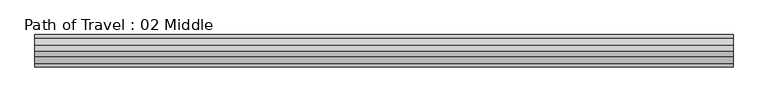
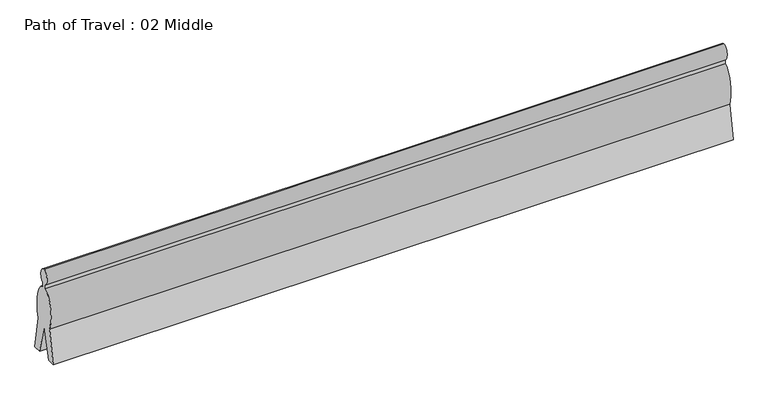
"""IFC4 building model written with IfcOpenShell, lengths in millimetres: proxy geometry, Path of Travel : 02 Middle."""

from ifc_helpers import new_model, si_unit, point, frame, origin, place, context, project, spatial, ellipse_curve, trimmed, source, transform, mapped, element, save
from ifc_brep_helpers import plane_surface, extruded_surface, advanced_brep


def path_of_travel_02_middle_47484a08(model_context):
    return source(origin(), model_context, "Body", "AdvancedBrep", [
        advanced_brep(
        [(227.5554837, 0.0, 1727.2), (227.5554837, 42.9018657, 1436.6534209), (227.5554837, 42.9018657, 1363.4763406), (227.5554837, 184.1186263, 643.4144547), (227.5554837, 297.5699544, 0.0), (227.5554837, 145.6574193, 0.0), (227.5554837, 0.0, 584.2), (227.5554837, -145.6574193, 0.0), (227.5554837, -297.5699544, 0.0), (227.5554837, -184.1186263, 643.4144547), (227.5554837, -42.9018657, 1363.4763406), (227.5554837, -42.9018657, 1436.6534209), (13029.1554837, 0.0, 1727.2), (13029.1554837, -42.9018657, 1436.6534209), (13029.1554837, -42.9018657, 1363.4763406), (13029.1554837, -184.1186263, 643.4144547), (13029.1554837, -297.5699544, 0.0), (13029.1554837, -145.6574193, 0.0), (13029.1554837, 0.0, 584.2), (13029.1554837, 145.6574193, 0.0), (13029.1554837, 297.5699544, 0.0), (13029.1554837, 184.1186263, 643.4144547), (13029.1554837, 42.9018657, 1363.4763406), (13029.1554837, 42.9018657, 1436.6534209)],
        [
            (0, 1, ellipse_curve(frame((227.5554837, 0.0, 1574.8), z_axis=(-1.0, 0.0, 0.0), x_axis=(0.0, 0.0, 1.0)), 152.4, 101.6)),
            (1, 2),
            (2, 3, ellipse_curve(frame((227.5554837, 0.0, 914.4), z_axis=(-1.0, 0.0, 0.0), x_axis=(0.0, 0.0, -1.0)), 457.2, 228.6)),
            (3, 4),
            (4, 5),
            (5, 6),
            (6, 7),
            (7, 8),
            (8, 9),
            (9, 10, ellipse_curve(frame((227.5554837, 0.0, 914.4), z_axis=(-1.0, 0.0, 0.0), x_axis=(0.0, 0.0, -1.0)), 457.2, 228.6)),
            (10, 11),
            (11, 0, ellipse_curve(frame((227.5554837, 0.0, 1574.8), z_axis=(-1.0, 0.0, 0.0), x_axis=(0.0, 0.0, 1.0)), 152.4, 101.6)),
            (12, 13, ellipse_curve(frame((13029.1554837, 0.0, 1574.8), z_axis=(1.0, 0.0, 0.0), x_axis=(0.0, 0.0, 1.0)), 152.4, 101.6)),
            (13, 14),
            (14, 15, ellipse_curve(frame((13029.1554837, 0.0, 914.4), z_axis=(1.0, 0.0, 0.0), x_axis=(0.0, 0.0, -1.0)), 457.2, 228.6)),
            (15, 16),
            (16, 17),
            (17, 18),
            (18, 19),
            (19, 20),
            (20, 21),
            (21, 22, ellipse_curve(frame((13029.1554837, 0.0, 914.4), z_axis=(1.0, 0.0, 0.0), x_axis=(0.0, 0.0, -1.0)), 457.2, 228.6)),
            (22, 23),
            (23, 12, ellipse_curve(frame((13029.1554837, 0.0, 1574.8), z_axis=(1.0, 0.0, 0.0), x_axis=(0.0, 0.0, 1.0)), 152.4, 101.6)),
            (0, 12),
            (23, 1),
            (22, 2),
            (21, 3),
            (20, 4),
            (19, 5),
            (18, 6),
            (17, 7),
            (16, 8),
            (15, 9),
            (14, 10),
            (13, 11),
        ],
        [
            plane_surface(frame((227.5554837, 0.0, 0.0), z_axis=(-1.0, 0.0, 0.0), x_axis=(0.0, 0.0, 1.0))),
            plane_surface(frame((13029.1554837, 0.0, 0.0), z_axis=(1.0, 0.0, 0.0), x_axis=(0.0, 0.0, 1.0))),
            extruded_surface(trimmed(ellipse_curve(frame((13029.1554837, 0.0, 1574.8), z_axis=(-1.0, 0.0, 0.0), x_axis=(0.0, 0.0, 1.0)), 152.4, 101.6), [point((13029.1554837, 0.0, 1727.2))], [point((13029.1554837, 42.9018657, 1436.6534209))], True, "CARTESIAN"), (-12801.6, 0.0, 0.0), 12801.6),
            plane_surface(frame((227.5554837, 42.9018657, 1436.6534209), z_axis=(0.0, 1.0, 0.0), x_axis=(1.0, 0.0, 0.0))),
            extruded_surface(trimmed(ellipse_curve(frame((13029.1554837, 0.0, 914.4), z_axis=(-1.0, 0.0, 0.0), x_axis=(0.0, 0.0, -1.0)), 457.2, 228.6), [point((13029.1554837, 42.9018657, 1363.4763406))], [point((13029.1554837, 184.1186263, 643.4144547))], True, "CARTESIAN"), (-12801.6, 0.0, 0.0), 12801.6),
            plane_surface(frame((227.5554837, 184.1186263, 643.4144547), z_axis=(0.0, 0.9848077530122078, 0.17364817766693205), x_axis=(1.0, 0.0, 0.0))),
            plane_surface(frame((227.5554837, 297.5699544, 0.0), z_axis=(0.0, 0.0, -1.0), x_axis=(1.0, 0.0, 0.0))),
            plane_surface(frame((227.5554837, 145.6574193, 0.0), z_axis=(0.0, -0.9702957262760199, -0.2419218955995739), x_axis=(1.0, 0.0, 0.0))),
            plane_surface(frame((227.5554837, 0.0, 584.2), z_axis=(0.0, 0.9702957262759961, -0.24192189559966923), x_axis=(1.0, 0.0, 0.0))),
            plane_surface(frame((227.5554837, -145.6574193, 0.0), z_axis=(0.0, 0.0, -1.0), x_axis=(1.0, 0.0, 0.0))),
            plane_surface(frame((227.5554837, -297.5699544, 0.0), z_axis=(0.0, -0.984807753012208, 0.17364817766693066), x_axis=(1.0, 0.0, 0.0))),
            extruded_surface(trimmed(ellipse_curve(frame((13029.1554837, 0.0, 914.4), z_axis=(-1.0, 0.0, 0.0), x_axis=(0.0, 0.0, -1.0)), 457.2, 228.6), [point((13029.1554837, -184.1186263, 643.4144547))], [point((13029.1554837, -42.9018657, 1363.4763406))], True, "CARTESIAN"), (-12801.6, 0.0, 0.0), 12801.6),
            plane_surface(frame((227.5554837, -42.9018657, 1363.4763406), z_axis=(0.0, -1.0, 0.0), x_axis=(1.0, 0.0, 0.0))),
            extruded_surface(trimmed(ellipse_curve(frame((13029.1554837, 0.0, 1574.8), z_axis=(-1.0, 0.0, 0.0), x_axis=(0.0, 0.0, 1.0)), 152.4, 101.6), [point((13029.1554837, -42.9018657, 1436.6534209))], [point((13029.1554837, 0.0, 1727.2))], True, "CARTESIAN"), (-12801.6, 0.0, 0.0), 12801.6),
        ],
        [
            (0, [[1, 2, 3, 4, 5, 6, 7, 8, 9, 10, 11, 12]]),
            (1, [[13, 14, 15, 16, 17, 18, 19, 20, 21, 22, 23, 24]]),
            (2, [[-1, 25, -24, 26]]),
            (3, [[-2, -26, -23, 27]]),
            (4, [[-3, -27, -22, 28]]),
            (5, [[-4, -28, -21, 29]]),
            (6, [[-5, -29, -20, 30]]),
            (7, [[-6, -30, -19, 31]]),
            (8, [[-7, -31, -18, 32]]),
            (9, [[-8, -32, -17, 33]]),
            (10, [[-9, -33, -16, 34]]),
            (11, [[-10, -34, -15, 35]]),
            (12, [[-11, -35, -14, 36]]),
            (13, [[-12, -36, -13, -25]]),
        ],
    ),
    ])


if __name__ == "__main__":
    model = new_model("IFC4")
    model_context = context("Model", 3, world=origin())
    ifc_project = project(units=[si_unit("LENGTHUNIT", "METRE", prefix="MILLI")], contexts=[model_context])
    site = spatial("IfcSite", under=ifc_project)
    building = spatial("IfcBuilding", under=site)
    placement = place(None, origin())
    path_of_travel_02_middle_shape = path_of_travel_02_middle_47484a08(model_context)
    element("IfcBuildingElementProxy", 1, Name="Path of Travel : 02 Middle", ObjectType="Path of Travel : 02 Middle", at=placement, inside=building, context=model_context, shape_type="MappedRepresentation", body=[
        mapped(path_of_travel_02_middle_shape, transform((0.0, 0.0, 0.0), x_axis=(1.0, 0.0, 0.0), y_axis=(0.0, 1.0, 0.0), z_axis=(0.0, 0.0, 1.0))),
    ])
    save(model, "model.ifc")

# Revit data of these elements
# Type "Path of Travel : 02 Middle"
#   Path of Egress [instance default] = 4' - 0"
#   built-in parameter 1001306 [instance default] = 4 (stored number, unit not read)
#   Dot at Start = no
#   Arrow in Middle = yes
#   Arrow at End = no
#   Egress Path = none
# Element 1 (IfcBuildingElementProxy, "Path of Travel : 02 Middle")
#   Path of Egress = 42' - 0"
#   built-in parameter 1001306 = 42 (stored number, unit not read)
#   Materials on its faces: "Egress Path Solid"
# Materials
#   "Egress Path Solid": class "Unassigned", colour RGB 255 128 64, transparency 0.75, Comments = "Rendering appearance not upgraded "
